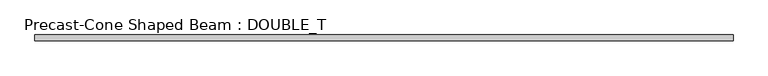
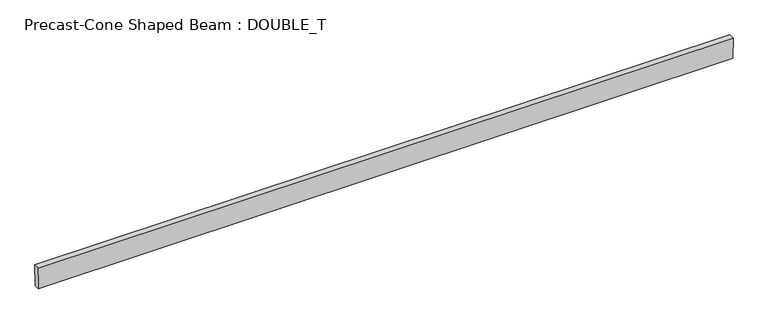
"""IFC4 building model written with IfcOpenShell, lengths in millimetres: beam geometry, Precast-Cone Shaped Beam : DOUBLE_T."""

import ifcopenshell
import ifcopenshell.guid

model = None  # the IFC model being written
_history = None  # IfcOwnerHistory: only IFC2X3 demands one
_inside = {}  # id of a spatial element -> (the spatial element, [elements in it])
_under = {}  # id of a project, library or spatial element -> (it, [spatial elements below it])
_declared = {}  # id of a project -> (the project, [libraries it declares])
_typed = {}  # id of a type object -> (the type object, [elements of that type])
_made_of = {}  # id of a material, layer set ... -> (it, [elements and type objects made of it])


def new_model(schema):
    """Start an empty IFC model of exactly this schema.

    Asked for "IFC4X3", IfcOpenShell would pick the latest addendum, in which some entities
    have other attributes; the version numbers below select the first issue.
    IFC2X3 requires an IfcOwnerHistory on every rooted entity: one is made here for all.
    """
    global model, _history
    if schema == "IFC4X3":
        model = ifcopenshell.file(schema_version=(4, 3, 0, 0))
    else:
        model = ifcopenshell.file(schema=schema)
    _inside.clear()
    _under.clear()
    _declared.clear()
    _typed.clear()
    _made_of.clear()
    _history = None
    if model.schema == "IFC2X3":
        org = make("IfcOrganization", Name="unknown")
        user = make(
            "IfcPersonAndOrganization",
            ThePerson=make("IfcPerson", FamilyName="unknown"),
            TheOrganization=org,
        )
        app = make(
            "IfcApplication",
            ApplicationDeveloper=org,
            Version="unknown",
            ApplicationFullName="unknown",
            ApplicationIdentifier="unknown",
        )
        _history = make(
            "IfcOwnerHistory",
            OwningUser=user,
            OwningApplication=app,
            ChangeAction="ADDED",
            CreationDate=0,
        )
    return model


def make(cls, **values):
    """One entity of the class cls with the attributes given. An attribute that is None is left unset."""
    return model.create_entity(
        cls, **{name: value for name, value in values.items() if value is not None}
    )


def rooted(cls, **values):
    """An entity with a GlobalId (a new one), such as an element, a storey or a relation."""
    return make(cls, GlobalId=ifcopenshell.guid.new(), OwnerHistory=_history, **values)


def si_unit(unit_type, name, prefix=None):
    """IfcSIUnit, for example si_unit("LENGTHUNIT", "METRE", prefix="MILLI")."""
    return make("IfcSIUnit", UnitType=unit_type, Prefix=prefix, Name=name)


def assignment(units):
    """IfcUnitAssignment: the units of a project."""
    return None if units is None else make("IfcUnitAssignment", Units=units)


def point(xyz):
    """IfcCartesianPoint."""
    return None if xyz is None else make("IfcCartesianPoint", Coordinates=xyz)


def direction(xyz):
    """IfcDirection."""
    return None if xyz is None else make("IfcDirection", DirectionRatios=xyz)


def frame(location, z_axis=None, x_axis=None):
    """IfcAxis2Placement3D, a coordinate frame: its origin and axes. An axis left out is left unset."""
    return make(
        "IfcAxis2Placement3D",
        Location=point(location),
        Axis=direction(z_axis),
        RefDirection=direction(x_axis),
    )


def origin():
    """The frame at (0, 0, 0) with its axes left unset."""
    return frame((0.0, 0.0, 0.0))


def place(relative_to, where):
    """IfcLocalPlacement: puts the frame where relative to a parent placement (None: the world)."""
    return make(
        "IfcLocalPlacement", PlacementRelTo=relative_to, RelativePlacement=where
    )


def context(
    kind, dimensions, precision=None, world=None, true_north=None, identifier=None
):
    """IfcGeometricRepresentationContext, for example the 3D "Model" context."""
    return make(
        "IfcGeometricRepresentationContext",
        ContextIdentifier=identifier,
        ContextType=kind,
        CoordinateSpaceDimension=dimensions,
        Precision=precision,
        WorldCoordinateSystem=world,
        TrueNorth=true_north,
    )


def project(units=None, contexts=None):
    """IfcProject with its units and contexts."""
    return rooted(
        "IfcProject",
        Name="project",
        RepresentationContexts=contexts,
        UnitsInContext=assignment(units),
    )


def spatial(cls, under=None, at=None, **own):
    """A site, building, storey or space (cls), placed at a placement, below another one or the project."""
    s = rooted(cls, ObjectPlacement=at, **own)
    if under is not None:
        _under.setdefault(under.id(), (under, []))[1].append(s)
    return s


def polyline(points):
    """IfcPolyline through the points."""
    return make("IfcPolyline", Points=[point(p) for p in points])


def outline(outer, holes=None, kind="AREA"):
    """IfcArbitraryClosedProfileDef: a profile drawn as a closed curve; with holes, ...WithVoids."""
    if holes is None:
        return make("IfcArbitraryClosedProfileDef", ProfileType=kind, OuterCurve=outer)
    return make(
        "IfcArbitraryProfileDefWithVoids",
        ProfileType=kind,
        OuterCurve=outer,
        InnerCurves=holes,
    )


def extrude(swept, where, along, depth):
    """IfcExtrudedAreaSolid: the profile swept, set in the frame where, extruded along a direction by depth."""
    return make(
        "IfcExtrudedAreaSolid",
        SweptArea=swept,
        Position=where,
        ExtrudedDirection=direction(along),
        Depth=depth,
    )


def shape(context_of_items, identifier, shape_type, items):
    """IfcShapeRepresentation: the items that make up one representation, for example the "Body"."""
    return make(
        "IfcShapeRepresentation",
        ContextOfItems=context_of_items,
        RepresentationIdentifier=identifier,
        RepresentationType=shape_type,
        Items=items,
    )


def source(mapping_origin, context_of_items, identifier, shape_type, items):
    """IfcRepresentationMap: a shape defined once, which mapped items show again and again."""
    return make(
        "IfcRepresentationMap",
        MappingOrigin=mapping_origin,
        MappedRepresentation=shape(context_of_items, identifier, shape_type, items),
    )


def transform(
    local_origin,
    x_axis=None,
    y_axis=None,
    z_axis=None,
    scale=None,
    scale2=None,
    scale3=None,
    uniform=True,
):
    """IfcCartesianTransformationOperator3D, or its non-uniform kind. x_axis, y_axis, z_axis: its Axis1, 2, 3."""
    if uniform:
        return make(
            "IfcCartesianTransformationOperator3D",
            Axis1=direction(x_axis),
            Axis2=direction(y_axis),
            LocalOrigin=point(local_origin),
            Scale=scale,
            Axis3=direction(z_axis),
        )
    return make(
        "IfcCartesianTransformationOperator3DnonUniform",
        Axis1=direction(x_axis),
        Axis2=direction(y_axis),
        LocalOrigin=point(local_origin),
        Scale=scale,
        Axis3=direction(z_axis),
        Scale2=scale2,
        Scale3=scale3,
    )


def mapped(mapping_source, mapping_target):
    """IfcMappedItem: shows the shape of a source again, moved by a transform."""
    return make(
        "IfcMappedItem", MappingSource=mapping_source, MappingTarget=mapping_target
    )


def made_of(thing, what):
    """Note that an element or type object is made of a material, layer set ...; save() writes the relation."""
    if what is not None:
        _made_of.setdefault(what.id(), (what, []))[1].append(thing)
    return thing


def element(
    cls,
    number,
    at=None,
    inside=None,
    cuts=None,
    type_object=None,
    material=None,
    context=None,
    identifier="Body",
    shape_type=None,
    held_by="IfcProductDefinitionShape",
    body=None,
    shapes=None,
    **own,
):
    """One element of the class cls, such as IfcWall. Its Tag is "e" and its number.

    at: its placement. inside: the storey or other place that contains it. cuts: it is an
    opening in that element (IfcRelVoidsElement). A single representation is given by context,
    identifier, shape_type and body (its items); several are given by shapes. held_by: the class
    of the entity that holds the representations. save() writes the other relations.
    """
    e = rooted(cls, Tag="e%d" % number, ObjectPlacement=at, **own)
    if body is not None:
        shapes = [shape(context, identifier, shape_type, body)]
    if shapes is not None:
        e.Representation = make(held_by, Representations=shapes)
    if inside is not None:
        _inside.setdefault(inside.id(), (inside, []))[1].append(e)
    if cuts is not None:
        rooted(
            "IfcRelVoidsElement", RelatingBuildingElement=cuts, RelatedOpeningElement=e
        )
    if type_object is not None:
        _typed.setdefault(type_object.id(), (type_object, []))[1].append(e)
    return made_of(e, material)


def aggregate(whole, parts):
    """IfcRelAggregates: a whole, such as a stair, and the parts it consists of."""
    return rooted("IfcRelAggregates", RelatingObject=whole, RelatedObjects=parts)


def save(model, path):
    """Write the relations noted so far, then the file.

    IfcRelAggregates (storeys below a building ...), IfcRelContainedInSpatialStructure (elements
    in a storey), IfcRelDefinesByType, IfcRelAssociatesMaterial and IfcRelDeclares: one each for
    every whole, place, type object, material and project.
    """
    for whole, parts in _under.values():
        aggregate(whole, parts)
    for where, things in _inside.values():
        rooted(
            "IfcRelContainedInSpatialStructure",
            RelatedElements=things,
            RelatingStructure=where,
        )
    for kind, things in _typed.values():
        rooted("IfcRelDefinesByType", RelatedObjects=things, RelatingType=kind)
    for what, things in _made_of.values():
        rooted("IfcRelAssociatesMaterial", RelatedObjects=things, RelatingMaterial=what)
    for by, libraries in _declared.values():
        rooted("IfcRelDeclares", RelatingContext=by, RelatedDefinitions=libraries)
    model.write(path)


def precast_cone_shaped_beam_double_t_e9a1f935(model_context):
    return source(origin(), model_context, "Body", "SweptSolid", [
        extrude(outline(polyline([(50.8, -228.6), (-50.8, -228.6), (-63.5, 228.6), (63.5, 228.6), (50.8, -228.6)])), frame((-7162.8, 0.0, 0.0), z_axis=(1.0, 0.0, 0.0), x_axis=(0.0, 1.0, 0.0)), (0.0, 0.0, 1.0), 14693.9),
    ])


if __name__ == "__main__":
    model = new_model("IFC4")
    model_context = context("Model", 3, world=origin())
    ifc_project = project(units=[si_unit("LENGTHUNIT", "METRE", prefix="MILLI")], contexts=[model_context])
    site = spatial("IfcSite", under=ifc_project)
    building = spatial("IfcBuilding", under=site)
    placement = place(None, origin())
    precast_cone_shaped_beam_double_t_shape = precast_cone_shaped_beam_double_t_e9a1f935(model_context)
    element("IfcBeam", 1, ObjectType="Precast-Cone Shaped Beam : DOUBLE_T", at=placement, inside=building, context=model_context, shape_type="MappedRepresentation", body=[
        mapped(precast_cone_shaped_beam_double_t_shape, transform((0.0, 0.0, 0.0), x_axis=(1.0, 0.0, 0.0), y_axis=(0.0, 1.0, 0.0), z_axis=(0.0, 0.0, 1.0))),
    ])
    save(model, "model.ifc")

# Revit data of these elements
# Type "Precast-Cone Shaped Beam : DOUBLE_T"
#   Top Width = 0' - 5"
#   Tie Rod Weight [instance default] = 30
#   Tie Rod W [instance default] = 0.0660938 kip
#   Single Rebar Weight [instance default] = 50
#   Single Rebar W [instance default] = 0.110156 kip
#   Rebar Grids Weight [instance default] = 100
#   Rebar Grids W [instance default] = 0.220313 kip
#   Depth = 1' - 6"
#   Bottom Width = 0' - 4"
#   Length [instance default] = 5' - 0"
#   Structural Material [instance default] = Concrete, Precast
#   Assembly Code = ""
# Element 1 (IfcBeam, "Precast-Cone Shaped Beam : DOUBLE_T")
#   Length = 49' - 5"
#   Structural Material = Concrete - Precast Concrete - Normal Weight Concrete - 5 ksi
#   Materials on its faces: "Concrete - Precast Concrete - Normal Weight Concrete - 5 ksi"
# Materials
#   "Concrete, Precast": class "Concrete", colour RGB 198 187 187, transparency 0, Description = "Precast concrete", Cost = 0
#   "Concrete - Precast Concrete - Normal Weight Concrete - 5 ksi": class "Concrete", colour RGB 198 187 187, transparency 0, Cost = 0
